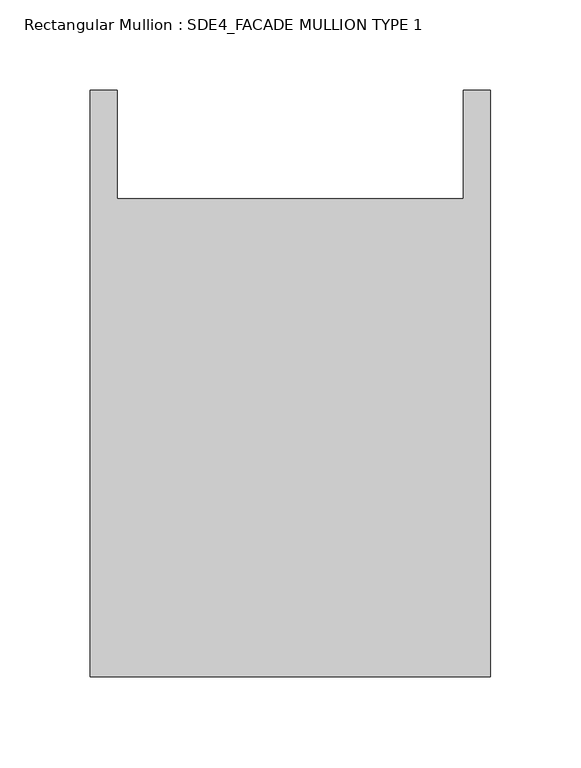
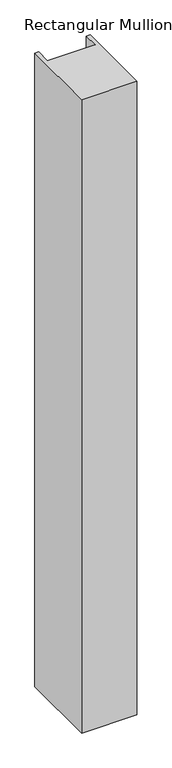
"""IFC4 building model written with IfcOpenShell, lengths in millimetres: member geometry, Rectangular Mullion : SDE4_FACADE MULLION TYPE 1."""

from ifc_helpers import new_model, si_unit, frame, origin, place, context, project, spatial, polyline, outline, extrude, source, transform, mapped, element, save


def rectangular_mullion_sde4_facade_mullion_type_1_749a7d1c(model_context):
    return source(origin(), model_context, "Body", "SweptSolid", [
        extrude(outline(polyline([(111.0, -132.5), (-111.0, -132.5), (-111.0, 192.5), (-96.0, 192.5), (-96.0, 132.5), (96.0, 132.5), (96.0, 192.5), (111.0, 192.5), (111.0, -132.5)])), frame((0.0, 0.0, -2687.1714687), z_axis=(0.0, 0.0, 1.0), x_axis=(1.0, 0.0, 0.0)), (0.0, 0.0, 1.0), 2687.1714687),
    ])


if __name__ == "__main__":
    model = new_model("IFC4")
    model_context = context("Model", 3, world=origin())
    ifc_project = project(units=[si_unit("LENGTHUNIT", "METRE", prefix="MILLI")], contexts=[model_context])
    site = spatial("IfcSite", under=ifc_project)
    building = spatial("IfcBuilding", under=site)
    placement = place(None, origin())
    rectangular_mullion_sde4_facade_mullion_type_1_shape = rectangular_mullion_sde4_facade_mullion_type_1_749a7d1c(model_context)
    element("IfcMember", 1, ObjectType="Rectangular Mullion : SDE4_FACADE MULLION TYPE 1", at=placement, inside=building, context=model_context, shape_type="MappedRepresentation", body=[
        mapped(rectangular_mullion_sde4_facade_mullion_type_1_shape, transform((0.0, 0.0, 0.0), x_axis=(1.0, 0.0, 0.0), y_axis=(0.0, 1.0, 0.0), z_axis=(0.0, 0.0, 1.0))),
    ])
    save(model, "model.ifc")

# Revit data of these elements
# Type "Rectangular Mullion : SDE4_FACADE MULLION TYPE 1"
#   built-in parameter 1007322 = 0.869423 (stored number, unit not read)
#   built-in parameter 1007321 = 0.364173 (stored number, unit not read)
#   built-in parameter 1007320 = 0.364173 (stored number, unit not read)
